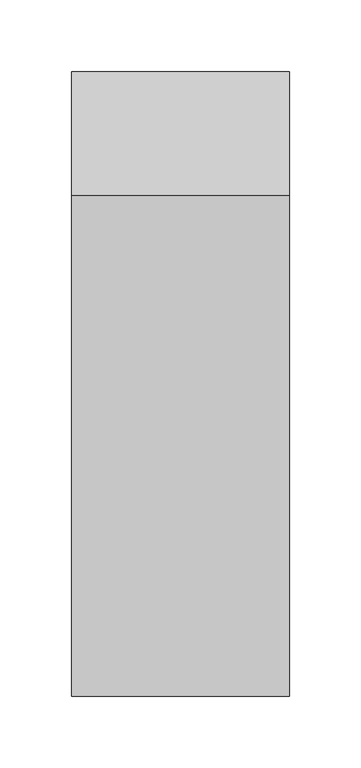
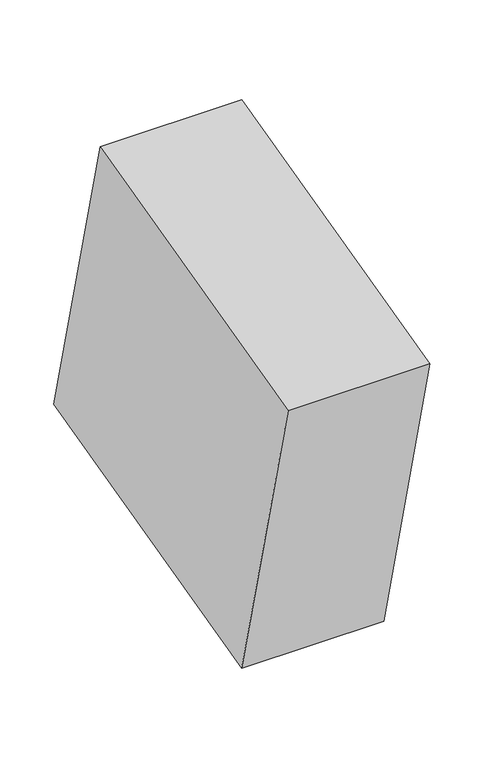
"""IFC4 building model written with IfcOpenShell, lengths in millimetres: proxy geometry, Framing019 3148 : Framing019 3148."""

from ifc_helpers import new_model, si_unit, frame, origin, place, context, project, spatial, polyline, outline, extrude, source, transform, mapped, element, save


def generic_models_88cac3fd(model_context):
    return source(origin(), model_context, "Body", "SweptSolid", [
        extrude(outline(polyline([(10616.8128942, 43457.8953321), (10266.6377213, 43370.3515388), (10180.3882058, 43715.2646709), (10530.5446077, 43802.8723498), (10616.8128942, 43457.8953321)])), frame((4322.6883192, 0.0, 0.0), z_axis=(1.0, 0.0, 0.0), x_axis=(0.0, 1.0, 0.0)), (0.0, 0.0, 1.0), 152.4),
    ])


if __name__ == "__main__":
    model = new_model("IFC4")
    model_context = context("Model", 3, world=origin())
    ifc_project = project(units=[si_unit("LENGTHUNIT", "METRE", prefix="MILLI")], contexts=[model_context])
    site = spatial("IfcSite", under=ifc_project)
    building = spatial("IfcBuilding", under=site)
    placement = place(None, origin())
    generic_models_shape = generic_models_88cac3fd(model_context)
    element("IfcBuildingElementProxy", 1, Name="Framing019 3148 : Framing019 3148", ObjectType="Framing019 3148 : Framing019 3148", at=placement, inside=building, context=model_context, shape_type="MappedRepresentation", body=[
        mapped(generic_models_shape, transform((0.0, 0.0, 0.0), x_axis=(1.0, 0.0, 0.0), y_axis=(0.0, 1.0, 0.0), z_axis=(0.0, 0.0, 1.0))),
    ])
    save(model, "model.ifc")

# Revit data of these elements
# Type "Framing019 3148 : Framing019 3148"
#   NameOverride = "Framing019"
# Element 1 (IfcBuildingElementProxy, "Framing019 3148 : Framing019 3148")
#   Materials on its faces: "WOOD FRAMING (SEE STRUCT DWGS)"
# Materials
#   "WOOD FRAMING (SEE STRUCT DWGS)": class "Unassigned", colour RGB 224 188 168, transparency 0, Cost = 0
